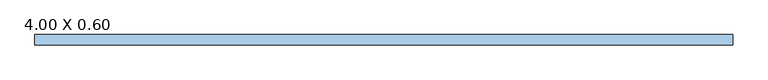
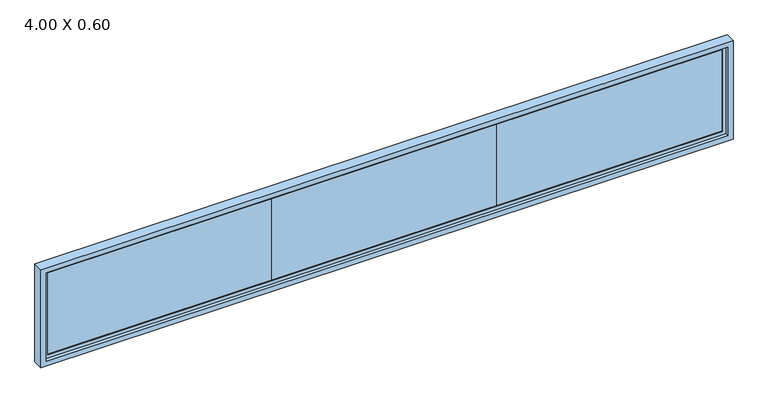
"""IFC4 building model written with IfcOpenShell, lengths in millimetres: window geometry, .CC_ND 300_JANELA FIXA_VIDRO : 4.00 X 0.60."""

import ifcopenshell
import ifcopenshell.guid

model = None  # the IFC model being written
_history = None  # IfcOwnerHistory: only IFC2X3 demands one
_inside = {}  # id of a spatial element -> (the spatial element, [elements in it])
_under = {}  # id of a project, library or spatial element -> (it, [spatial elements below it])
_declared = {}  # id of a project -> (the project, [libraries it declares])
_typed = {}  # id of a type object -> (the type object, [elements of that type])
_made_of = {}  # id of a material, layer set ... -> (it, [elements and type objects made of it])


def new_model(schema):
    """Start an empty IFC model of exactly this schema.

    Asked for "IFC4X3", IfcOpenShell would pick the latest addendum, in which some entities
    have other attributes; the version numbers below select the first issue.
    IFC2X3 requires an IfcOwnerHistory on every rooted entity: one is made here for all.
    """
    global model, _history
    if schema == "IFC4X3":
        model = ifcopenshell.file(schema_version=(4, 3, 0, 0))
    else:
        model = ifcopenshell.file(schema=schema)
    _inside.clear()
    _under.clear()
    _declared.clear()
    _typed.clear()
    _made_of.clear()
    _history = None
    if model.schema == "IFC2X3":
        org = make("IfcOrganization", Name="unknown")
        user = make(
            "IfcPersonAndOrganization",
            ThePerson=make("IfcPerson", FamilyName="unknown"),
            TheOrganization=org,
        )
        app = make(
            "IfcApplication",
            ApplicationDeveloper=org,
            Version="unknown",
            ApplicationFullName="unknown",
            ApplicationIdentifier="unknown",
        )
        _history = make(
            "IfcOwnerHistory",
            OwningUser=user,
            OwningApplication=app,
            ChangeAction="ADDED",
            CreationDate=0,
        )
    return model


def make(cls, **values):
    """One entity of the class cls with the attributes given. An attribute that is None is left unset."""
    return model.create_entity(
        cls, **{name: value for name, value in values.items() if value is not None}
    )


def rooted(cls, **values):
    """An entity with a GlobalId (a new one), such as an element, a storey or a relation."""
    return make(cls, GlobalId=ifcopenshell.guid.new(), OwnerHistory=_history, **values)


def si_unit(unit_type, name, prefix=None):
    """IfcSIUnit, for example si_unit("LENGTHUNIT", "METRE", prefix="MILLI")."""
    return make("IfcSIUnit", UnitType=unit_type, Prefix=prefix, Name=name)


def assignment(units):
    """IfcUnitAssignment: the units of a project."""
    return None if units is None else make("IfcUnitAssignment", Units=units)


def point(xyz):
    """IfcCartesianPoint."""
    return None if xyz is None else make("IfcCartesianPoint", Coordinates=xyz)


def direction(xyz):
    """IfcDirection."""
    return None if xyz is None else make("IfcDirection", DirectionRatios=xyz)


def frame(location, z_axis=None, x_axis=None):
    """IfcAxis2Placement3D, a coordinate frame: its origin and axes. An axis left out is left unset."""
    return make(
        "IfcAxis2Placement3D",
        Location=point(location),
        Axis=direction(z_axis),
        RefDirection=direction(x_axis),
    )


def origin():
    """The frame at (0, 0, 0) with its axes left unset."""
    return frame((0.0, 0.0, 0.0))


def place(relative_to, where):
    """IfcLocalPlacement: puts the frame where relative to a parent placement (None: the world)."""
    return make(
        "IfcLocalPlacement", PlacementRelTo=relative_to, RelativePlacement=where
    )


def context(
    kind, dimensions, precision=None, world=None, true_north=None, identifier=None
):
    """IfcGeometricRepresentationContext, for example the 3D "Model" context."""
    return make(
        "IfcGeometricRepresentationContext",
        ContextIdentifier=identifier,
        ContextType=kind,
        CoordinateSpaceDimension=dimensions,
        Precision=precision,
        WorldCoordinateSystem=world,
        TrueNorth=true_north,
    )


def project(units=None, contexts=None):
    """IfcProject with its units and contexts."""
    return rooted(
        "IfcProject",
        Name="project",
        RepresentationContexts=contexts,
        UnitsInContext=assignment(units),
    )


def spatial(cls, under=None, at=None, **own):
    """A site, building, storey or space (cls), placed at a placement, below another one or the project."""
    s = rooted(cls, ObjectPlacement=at, **own)
    if under is not None:
        _under.setdefault(under.id(), (under, []))[1].append(s)
    return s


def polyline(points):
    """IfcPolyline through the points."""
    return make("IfcPolyline", Points=[point(p) for p in points])


def outline(outer, holes=None, kind="AREA"):
    """IfcArbitraryClosedProfileDef: a profile drawn as a closed curve; with holes, ...WithVoids."""
    if holes is None:
        return make("IfcArbitraryClosedProfileDef", ProfileType=kind, OuterCurve=outer)
    return make(
        "IfcArbitraryProfileDefWithVoids",
        ProfileType=kind,
        OuterCurve=outer,
        InnerCurves=holes,
    )


def extrude(swept, where, along, depth):
    """IfcExtrudedAreaSolid: the profile swept, set in the frame where, extruded along a direction by depth."""
    return make(
        "IfcExtrudedAreaSolid",
        SweptArea=swept,
        Position=where,
        ExtrudedDirection=direction(along),
        Depth=depth,
    )


def shape(context_of_items, identifier, shape_type, items):
    """IfcShapeRepresentation: the items that make up one representation, for example the "Body"."""
    return make(
        "IfcShapeRepresentation",
        ContextOfItems=context_of_items,
        RepresentationIdentifier=identifier,
        RepresentationType=shape_type,
        Items=items,
    )


def source(mapping_origin, context_of_items, identifier, shape_type, items):
    """IfcRepresentationMap: a shape defined once, which mapped items show again and again."""
    return make(
        "IfcRepresentationMap",
        MappingOrigin=mapping_origin,
        MappedRepresentation=shape(context_of_items, identifier, shape_type, items),
    )


def transform(
    local_origin,
    x_axis=None,
    y_axis=None,
    z_axis=None,
    scale=None,
    scale2=None,
    scale3=None,
    uniform=True,
):
    """IfcCartesianTransformationOperator3D, or its non-uniform kind. x_axis, y_axis, z_axis: its Axis1, 2, 3."""
    if uniform:
        return make(
            "IfcCartesianTransformationOperator3D",
            Axis1=direction(x_axis),
            Axis2=direction(y_axis),
            LocalOrigin=point(local_origin),
            Scale=scale,
            Axis3=direction(z_axis),
        )
    return make(
        "IfcCartesianTransformationOperator3DnonUniform",
        Axis1=direction(x_axis),
        Axis2=direction(y_axis),
        LocalOrigin=point(local_origin),
        Scale=scale,
        Axis3=direction(z_axis),
        Scale2=scale2,
        Scale3=scale3,
    )


def mapped(mapping_source, mapping_target):
    """IfcMappedItem: shows the shape of a source again, moved by a transform."""
    return make(
        "IfcMappedItem", MappingSource=mapping_source, MappingTarget=mapping_target
    )


def made_of(thing, what):
    """Note that an element or type object is made of a material, layer set ...; save() writes the relation."""
    if what is not None:
        _made_of.setdefault(what.id(), (what, []))[1].append(thing)
    return thing


def element(
    cls,
    number,
    at=None,
    inside=None,
    cuts=None,
    type_object=None,
    material=None,
    context=None,
    identifier="Body",
    shape_type=None,
    held_by="IfcProductDefinitionShape",
    body=None,
    shapes=None,
    **own,
):
    """One element of the class cls, such as IfcWall. Its Tag is "e" and its number.

    at: its placement. inside: the storey or other place that contains it. cuts: it is an
    opening in that element (IfcRelVoidsElement). A single representation is given by context,
    identifier, shape_type and body (its items); several are given by shapes. held_by: the class
    of the entity that holds the representations. save() writes the other relations.
    """
    e = rooted(cls, Tag="e%d" % number, ObjectPlacement=at, **own)
    if body is not None:
        shapes = [shape(context, identifier, shape_type, body)]
    if shapes is not None:
        e.Representation = make(held_by, Representations=shapes)
    if inside is not None:
        _inside.setdefault(inside.id(), (inside, []))[1].append(e)
    if cuts is not None:
        rooted(
            "IfcRelVoidsElement", RelatingBuildingElement=cuts, RelatedOpeningElement=e
        )
    if type_object is not None:
        _typed.setdefault(type_object.id(), (type_object, []))[1].append(e)
    return made_of(e, material)


def aggregate(whole, parts):
    """IfcRelAggregates: a whole, such as a stair, and the parts it consists of."""
    return rooted("IfcRelAggregates", RelatingObject=whole, RelatedObjects=parts)


def save(model, path):
    """Write the relations noted so far, then the file.

    IfcRelAggregates (storeys below a building ...), IfcRelContainedInSpatialStructure (elements
    in a storey), IfcRelDefinesByType, IfcRelAssociatesMaterial and IfcRelDeclares: one each for
    every whole, place, type object, material and project.
    """
    for whole, parts in _under.values():
        aggregate(whole, parts)
    for where, things in _inside.values():
        rooted(
            "IfcRelContainedInSpatialStructure",
            RelatedElements=things,
            RelatingStructure=where,
        )
    for kind, things in _typed.values():
        rooted("IfcRelDefinesByType", RelatedObjects=things, RelatingType=kind)
    for what, things in _made_of.values():
        rooted("IfcRelAssociatesMaterial", RelatedObjects=things, RelatingMaterial=what)
    for by, libraries in _declared.values():
        rooted("IfcRelDeclares", RelatingContext=by, RelatedDefinitions=libraries)
    model.write(path)


def window_4_00_x_0_60_0b555443(model_context):
    return source(origin(), model_context, "Body", "SweptSolid", [
        extrude(outline(polyline([(650.0, -4.0), (650.0, 4.0), (1950.0, 4.0), (1950.0, -4.0), (650.0, -4.0)])), frame((0.0, 0.0, 1550.0), z_axis=(0.0, 0.0, 1.0), x_axis=(1.0, 0.0, 0.0)), (0.0, 0.0, 1.0), 500.0),
        extrude(outline(polyline([(-650.0, -4.0), (-650.0, 4.0), (650.0, 4.0), (650.0, -4.0), (-650.0, -4.0)])), frame((0.0, 0.0, 1550.0), z_axis=(0.0, 0.0, 1.0), x_axis=(1.0, 0.0, 0.0)), (0.0, 0.0, 1.0), 500.0),
        extrude(outline(polyline([(-1950.0, -4.0), (-1950.0, 4.0), (-650.0, 4.0), (-650.0, -4.0), (-1950.0, -4.0)])), frame((0.0, 0.0, 1550.0), z_axis=(0.0, 0.0, 1.0), x_axis=(1.0, 0.0, 0.0)), (0.0, 0.0, 1.0), 500.0),
        extrude(outline(polyline([(1530.0, 1970.0), (2070.0, 1970.0), (2070.0, -1970.0), (1530.0, -1970.0), (1530.0, 1970.0)]), holes=[polyline([(2050.0, 1950.0), (1550.0, 1950.0), (1550.0, -1950.0), (2050.0, -1950.0), (2050.0, 1950.0)])]), frame((0.0, -10.0, 0.0), z_axis=(0.0, 1.0, 0.0), x_axis=(0.0, 0.0, 1.0)), (0.0, 0.0, 1.0), 20.0),
        extrude(outline(polyline([(1500.0, 2000.0), (2100.0, 2000.0), (2100.0, -2000.0), (1500.0, -2000.0), (1500.0, 2000.0)]), holes=[polyline([(2070.0, 1970.0), (1530.0, 1970.0), (1530.0, -1970.0), (2070.0, -1970.0), (2070.0, 1970.0)])]), frame((0.0, -30.0, 0.0), z_axis=(0.0, 1.0, 0.0), x_axis=(0.0, 0.0, 1.0)), (0.0, 0.0, 1.0), 60.0),
    ])


if __name__ == "__main__":
    model = new_model("IFC4")
    model_context = context("Model", 3, world=origin())
    ifc_project = project(units=[si_unit("LENGTHUNIT", "METRE", prefix="MILLI")], contexts=[model_context])
    site = spatial("IfcSite", under=ifc_project)
    building = spatial("IfcBuilding", under=site)
    placement = place(None, origin())
    window_4_00_x_0_60_shape = window_4_00_x_0_60_0b555443(model_context)
    element("IfcWindow", 1, ObjectType=".CC_ND 300_JANELA FIXA_VIDRO : 4.00 X 0.60", at=placement, inside=building, context=model_context, shape_type="MappedRepresentation", body=[
        mapped(window_4_00_x_0_60_shape, transform((0.0, 0.0, 0.0), x_axis=(1.0, 0.0, 0.0), y_axis=(0.0, 1.0, 0.0), z_axis=(0.0, 0.0, 1.0))),
    ])
    save(model, "model.ifc")

# Revit data of these elements
# Type ".CC_ND 300_JANELA FIXA_VIDRO : 4.00 X 0.60"
#   Type Mark = "60"
#   Largura total vidro [instance default] = 0.90 m
#   Largura Painel [instance default] = 0.02 m
#   Largura Esquadria [instance default] = 0.06 m
#   Espessuras [instance default] = 0.05 m
#   Espessura Vidro [instance default] = 0.008 m
#   Espessura Painel [instance default] = 0.02 m
#   Espessura Esquadria [instance default] = 0.03 m
#   Height = 0.60 m
#   Altura-padrão do peitoril = 1.50 m
#   Width = 4.00 m
#   Vidro = .VIDRO GENÉRICO
#   Esquadria = .ALUMÍNIO COM PINTURA ELETROSTÁTICA BRANCA
#   Wall Closure = (empty or 0)
# Element 1 (IfcWindow, ".CC_ND 300_JANELA FIXA_VIDRO : 4.00 X 0.60")
#   Materials on its faces: ".ALUMÍNIO COM PINTURA ELETROSTÁTICA BRANCA", ".VIDRO GENÉRICO"
# Materials
#   ".VIDRO GENÉRICO": class ".CC_VIDRO", colour RGB 0 128 192, transparency 0.9, Description = "Vidro comum", Cost = 0
#   ".ALUMÍNIO COM PINTURA ELETROSTÁTICA BRANCA": class "CC_METAIS", colour RGB 241 241 241, transparency 0, Cost = 0
